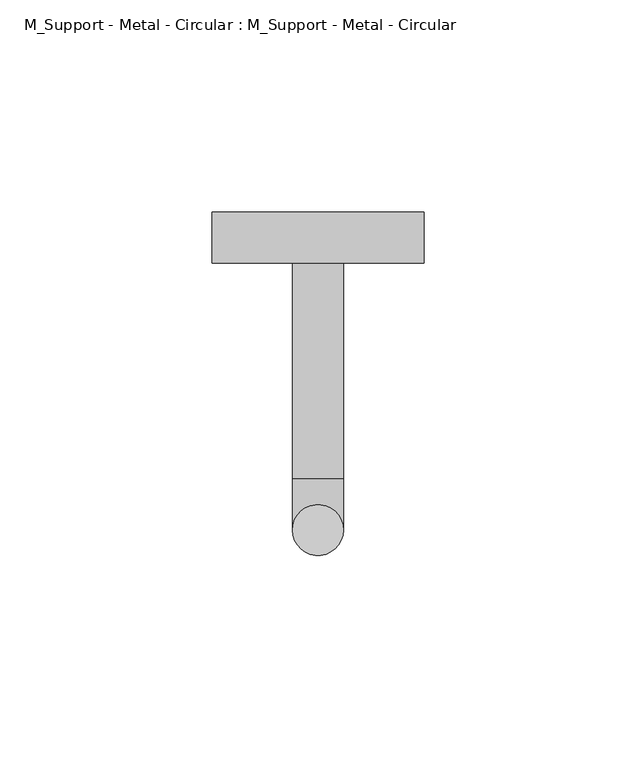
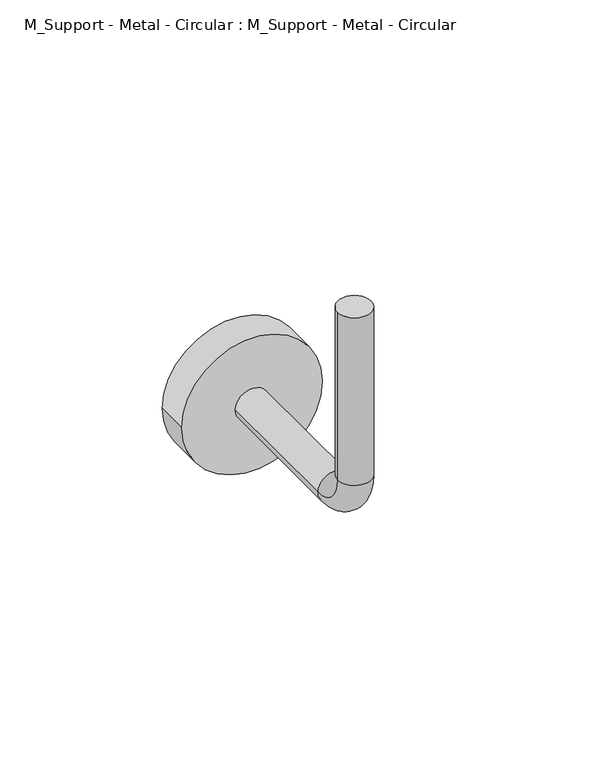
"""IFC4 building model written with IfcOpenShell, lengths in millimetres: proxy geometry, M_Support - Metal - Circular : M_Support - Metal - Circular."""

from ifc_helpers import new_model, si_unit, point, frame, frame_2d, origin, origin_with_axes, place, context, project, spatial, circle_curve, ellipse_curve, trimmed, segment, composite_curve, outline, extrude, source, transform, mapped, element, save
from ifc_brep_helpers import plane_surface, cylinder_surface, revolved_surface, advanced_brep


def m_support_metal_circular_m_support_metal_circular_a779fbb7(model_context):
    return source(origin(), model_context, "Body", "SolidModel", [
        advanced_brep(
        [(-6.0, 0.0, 0.0), (6.0, 0.0, 0.0), (-6.0, 0.0, -63.0), (6.0, 0.0, -63.0), (6.0, 12.0, -75.0), (-6.0, 12.0, -75.0), (-6.0, 63.0, -75.0), (6.0, 63.0, -75.0)],
        [
            (0, 1, circle_curve(origin_with_axes(), 6.0)),
            (1, 0, circle_curve(origin_with_axes(), 6.0)),
            (0, 2),
            (2, 3, circle_curve(frame((0.0, 0.0, -63.0), z_axis=(0.0, 0.0, 1.0), x_axis=(1.0, 0.0, 0.0)), 6.0)),
            (3, 1),
            (3, 2, circle_curve(frame((0.0, 0.0, -63.0), z_axis=(0.0, 0.0, 1.0), x_axis=(1.0, 0.0, 0.0)), 6.0)),
            (4, 3, circle_curve(frame((6.0, 12.0, -63.0), z_axis=(-1.0, 0.0, 0.0), x_axis=(0.0, -1.0, 0.0)), 12.0)),
            (2, 5, circle_curve(frame((-6.0, 12.0, -63.0), z_axis=(1.0, 0.0, 0.0), x_axis=(0.0, -1.0, 0.0)), 12.0)),
            (5, 4, circle_curve(frame((0.0, 12.0, -75.0), z_axis=(0.0, -1.0, 0.0), x_axis=(1.0, 0.0, 0.0)), 6.0)),
            (4, 5, circle_curve(frame((0.0, 12.0, -75.0), z_axis=(0.0, -1.0, 0.0), x_axis=(1.0, 0.0, 0.0)), 6.0)),
            (6, 7, circle_curve(frame((0.0, 63.0, -75.0), z_axis=(0.0, 1.0, 0.0), x_axis=(1.0, 0.0, 0.0)), 6.0)),
            (7, 6, circle_curve(frame((0.0, 63.0, -75.0), z_axis=(0.0, 1.0, 0.0), x_axis=(1.0, 0.0, 0.0)), 6.0)),
            (5, 6),
            (7, 4),
        ],
        [
            plane_surface(origin_with_axes()),
            cylinder_surface(origin_with_axes(), 6.0),
            revolved_surface(trimmed(ellipse_curve(frame((0.0, 0.0, -63.0), z_axis=(0.0, 0.0, 1.0), x_axis=(1.0, 0.0, 0.0)), 6.0, 6.0), [point((-6.0, 0.0, -63.0))], [point((6.0, 0.0, -63.0))], True, "CARTESIAN"), (0.0, 12.0, -63.0), (1.0, 0.0, 0.0)),
            revolved_surface(trimmed(ellipse_curve(frame((0.0, 0.0, -63.0), z_axis=(0.0, 0.0, 1.0), x_axis=(1.0, 0.0, 0.0)), 6.0, 6.0), [point((6.0, 0.0, -63.0))], [point((-6.0, 0.0, -63.0))], True, "CARTESIAN"), (0.0, 12.0, -63.0), (1.0, 0.0, 0.0)),
            plane_surface(frame((0.0, 63.0, -75.0), z_axis=(0.0, 1.0, 0.0), x_axis=(1.0, 0.0, 0.0))),
            cylinder_surface(frame((0.0, 12.0, -75.0), z_axis=(0.0, -1.0, 0.0), x_axis=(1.0, 0.0, 0.0)), 6.0),
        ],
        [
            (0, [[1, 2]]),
            (1, [[-1, 3, 4, 5]]),
            (1, [[-2, -5, 6, -3]]),
            (2, [[7, -4, 8, 9]]),
            (3, [[-8, -6, -7, 10]]),
            (4, [[11, 12]]),
            (5, [[-9, 13, -12, 14]]),
            (5, [[-10, -14, -11, -13]]),
        ],
    ),
        extrude(outline(composite_curve([segment(trimmed(circle_curve(frame_2d((-75.0, 0.0)), 25.0), [point((-75.0, -25.0))], [point((-75.0, 25.0))], False, "CARTESIAN"), True, "CONTINUOUS"), segment(trimmed(circle_curve(frame_2d((-75.0, 0.0)), 25.0), [point((-75.0, 25.0))], [point((-75.0, -25.0))], False, "CARTESIAN"), True, "CONTINUOUS")], self_intersect=False)), frame((0.0, 63.0, 0.0), z_axis=(0.0, 1.0, 0.0), x_axis=(0.0, 0.0, 1.0)), (0.0, 0.0, 1.0), 12.0),
    ])


if __name__ == "__main__":
    model = new_model("IFC4")
    model_context = context("Model", 3, world=origin())
    ifc_project = project(units=[si_unit("LENGTHUNIT", "METRE", prefix="MILLI")], contexts=[model_context])
    site = spatial("IfcSite", under=ifc_project)
    building = spatial("IfcBuilding", under=site)
    placement = place(None, origin())
    m_support_metal_circular_m_support_metal_circular_shape = m_support_metal_circular_m_support_metal_circular_a779fbb7(model_context)
    element("IfcBuildingElementProxy", 1, Name="M_Support - Metal - Circular : M_Support - Metal - Circular", ObjectType="M_Support - Metal - Circular : M_Support - Metal - Circular", at=placement, inside=building, context=model_context, shape_type="MappedRepresentation", body=[
        mapped(m_support_metal_circular_m_support_metal_circular_shape, transform((0.0, 0.0, 0.0), x_axis=(1.0, 0.0, 0.0), y_axis=(0.0, 1.0, 0.0), z_axis=(0.0, 0.0, 1.0))),
    ])
    save(model, "model.ifc")

# Revit data of these elements
# Type "M_Support - Metal - Circular : M_Support - Metal - Circular"
#   T1 = 12 mm
#   Radius 2 = 6 mm
#   Radius 1 = 25 mm
#   built-in parameter 1152166 = 0.246063 (stored number, unit not read)
#   built-in parameter 1152165 [instance default] = 0.246063 (stored number, unit not read)
#   Bend Radius = 12 mm
#   Support Material = Aluminum
# Element 1 (IfcBuildingElementProxy, "M_Support - Metal - Circular : M_Support - Metal - Circular")
#   Materials on its faces: "Aluminum"
# Materials
#   "Aluminum": class "Metal", colour RGB 247 247 247, transparency 0, Description = "Aluminum 6061", Cost = 0
